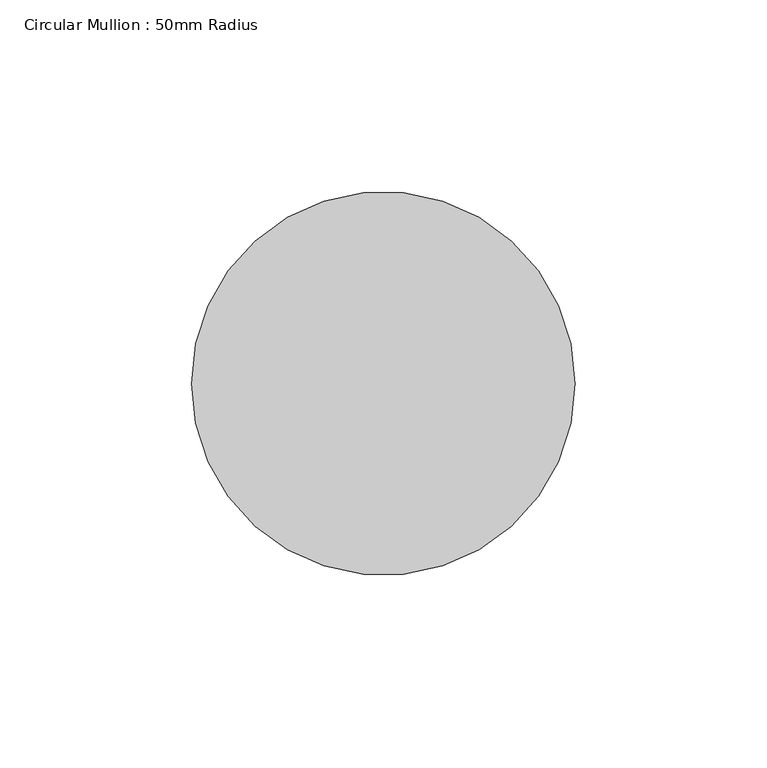
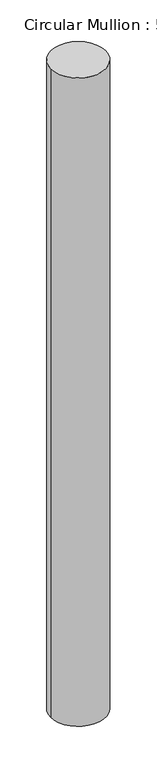
"""IFC4 building model written with IfcOpenShell, lengths in millimetres: member geometry, Circular Mullion : 50mm Radius."""

from ifc_helpers import new_model, si_unit, point, frame, origin, origin_2d, place, context, project, spatial, circle_curve, trimmed, segment, composite_curve, outline, extrude, source, transform, mapped, element, save


def circular_mullion_50mm_radius_3cf96d21(model_context):
    return source(origin(), model_context, "Body", "SweptSolid", [
        extrude(outline(composite_curve([segment(trimmed(circle_curve(origin_2d(), 50.0), [point((50.0, 0.0))], [point((-50.0, 0.0))], False, "CARTESIAN"), True, "CONTINUOUS"), segment(trimmed(circle_curve(origin_2d(), 50.0), [point((-50.0, 0.0))], [point((50.0, 0.0))], False, "CARTESIAN"), True, "CONTINUOUS")], self_intersect=False)), frame((0.0, 0.0, -1246.8647033), z_axis=(0.0, 0.0, 1.0), x_axis=(1.0, 0.0, 0.0)), (0.0, 0.0, 1.0), 1246.8647033),
    ])


if __name__ == "__main__":
    model = new_model("IFC4")
    model_context = context("Model", 3, world=origin())
    ifc_project = project(units=[si_unit("LENGTHUNIT", "METRE", prefix="MILLI")], contexts=[model_context])
    site = spatial("IfcSite", under=ifc_project)
    building = spatial("IfcBuilding", under=site)
    placement = place(None, origin())
    circular_mullion_50mm_radius_shape = circular_mullion_50mm_radius_3cf96d21(model_context)
    element("IfcMember", 1, ObjectType="Circular Mullion : 50mm Radius", at=placement, inside=building, context=model_context, shape_type="MappedRepresentation", body=[
        mapped(circular_mullion_50mm_radius_shape, transform((0.0, 0.0, 0.0), x_axis=(1.0, 0.0, 0.0), y_axis=(0.0, 1.0, 0.0), z_axis=(0.0, 0.0, 1.0))),
    ])
    save(model, "model.ifc")

# Revit data of these elements
# Type "Circular Mullion : 50mm Radius"
#   built-in parameter 1007350 = 0.164042 (stored number, unit not read)
# Element 1 (IfcMember, "Circular Mullion : 50mm Radius")
#   Materials on its faces: "Aluminium"
# Materials
#   "Aluminium": class "Metal", colour RGB 247 247 247, transparency 0, Description = "Aluminium 6061", Cost = 0
